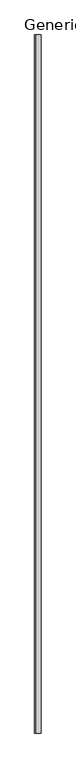
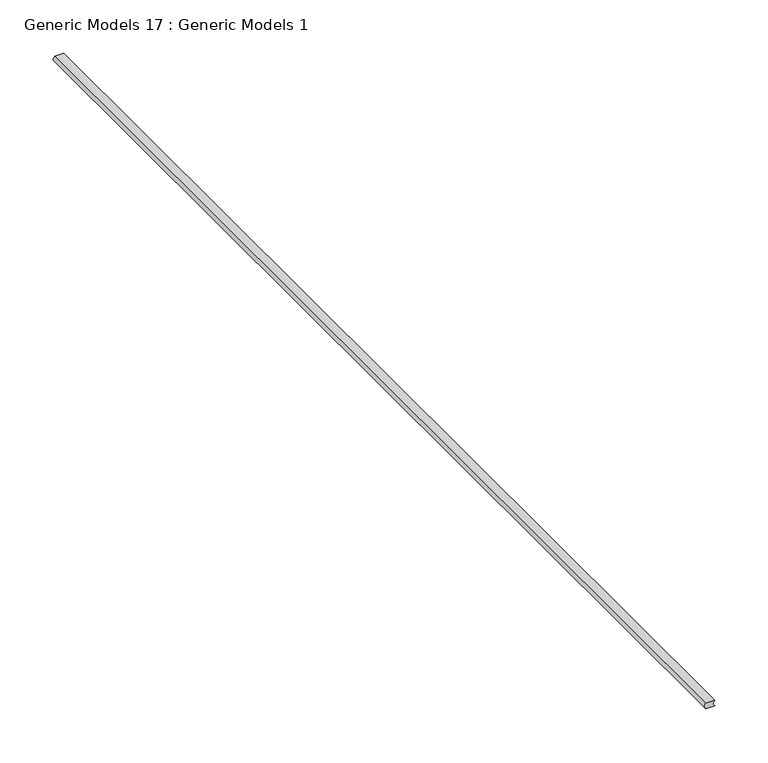
"""IFC4 building model written with IfcOpenShell, lengths in millimetres: proxy geometry, Generic Models 17 : Generic Models 1."""

import ifcopenshell
import ifcopenshell.guid

model = None  # the IFC model being written
_history = None  # IfcOwnerHistory: only IFC2X3 demands one
_inside = {}  # id of a spatial element -> (the spatial element, [elements in it])
_under = {}  # id of a project, library or spatial element -> (it, [spatial elements below it])
_declared = {}  # id of a project -> (the project, [libraries it declares])
_typed = {}  # id of a type object -> (the type object, [elements of that type])
_made_of = {}  # id of a material, layer set ... -> (it, [elements and type objects made of it])


def new_model(schema):
    """Start an empty IFC model of exactly this schema.

    Asked for "IFC4X3", IfcOpenShell would pick the latest addendum, in which some entities
    have other attributes; the version numbers below select the first issue.
    IFC2X3 requires an IfcOwnerHistory on every rooted entity: one is made here for all.
    """
    global model, _history
    if schema == "IFC4X3":
        model = ifcopenshell.file(schema_version=(4, 3, 0, 0))
    else:
        model = ifcopenshell.file(schema=schema)
    _inside.clear()
    _under.clear()
    _declared.clear()
    _typed.clear()
    _made_of.clear()
    _history = None
    if model.schema == "IFC2X3":
        org = make("IfcOrganization", Name="unknown")
        user = make(
            "IfcPersonAndOrganization",
            ThePerson=make("IfcPerson", FamilyName="unknown"),
            TheOrganization=org,
        )
        app = make(
            "IfcApplication",
            ApplicationDeveloper=org,
            Version="unknown",
            ApplicationFullName="unknown",
            ApplicationIdentifier="unknown",
        )
        _history = make(
            "IfcOwnerHistory",
            OwningUser=user,
            OwningApplication=app,
            ChangeAction="ADDED",
            CreationDate=0,
        )
    return model


def make(cls, **values):
    """One entity of the class cls with the attributes given. An attribute that is None is left unset."""
    return model.create_entity(
        cls, **{name: value for name, value in values.items() if value is not None}
    )


def rooted(cls, **values):
    """An entity with a GlobalId (a new one), such as an element, a storey or a relation."""
    return make(cls, GlobalId=ifcopenshell.guid.new(), OwnerHistory=_history, **values)


def si_unit(unit_type, name, prefix=None):
    """IfcSIUnit, for example si_unit("LENGTHUNIT", "METRE", prefix="MILLI")."""
    return make("IfcSIUnit", UnitType=unit_type, Prefix=prefix, Name=name)


def assignment(units):
    """IfcUnitAssignment: the units of a project."""
    return None if units is None else make("IfcUnitAssignment", Units=units)


def point(xyz):
    """IfcCartesianPoint."""
    return None if xyz is None else make("IfcCartesianPoint", Coordinates=xyz)


def direction(xyz):
    """IfcDirection."""
    return None if xyz is None else make("IfcDirection", DirectionRatios=xyz)


def frame(location, z_axis=None, x_axis=None):
    """IfcAxis2Placement3D, a coordinate frame: its origin and axes. An axis left out is left unset."""
    return make(
        "IfcAxis2Placement3D",
        Location=point(location),
        Axis=direction(z_axis),
        RefDirection=direction(x_axis),
    )


def frame_2d(location, x_axis=None):
    """IfcAxis2Placement2D, a coordinate frame in the plane: its origin and x axis."""
    return make(
        "IfcAxis2Placement2D", Location=point(location), RefDirection=direction(x_axis)
    )


def origin():
    """The frame at (0, 0, 0) with its axes left unset."""
    return frame((0.0, 0.0, 0.0))


def place(relative_to, where):
    """IfcLocalPlacement: puts the frame where relative to a parent placement (None: the world)."""
    return make(
        "IfcLocalPlacement", PlacementRelTo=relative_to, RelativePlacement=where
    )


def context(
    kind, dimensions, precision=None, world=None, true_north=None, identifier=None
):
    """IfcGeometricRepresentationContext, for example the 3D "Model" context."""
    return make(
        "IfcGeometricRepresentationContext",
        ContextIdentifier=identifier,
        ContextType=kind,
        CoordinateSpaceDimension=dimensions,
        Precision=precision,
        WorldCoordinateSystem=world,
        TrueNorth=true_north,
    )


def project(units=None, contexts=None):
    """IfcProject with its units and contexts."""
    return rooted(
        "IfcProject",
        Name="project",
        RepresentationContexts=contexts,
        UnitsInContext=assignment(units),
    )


def spatial(cls, under=None, at=None, **own):
    """A site, building, storey or space (cls), placed at a placement, below another one or the project."""
    s = rooted(cls, ObjectPlacement=at, **own)
    if under is not None:
        _under.setdefault(under.id(), (under, []))[1].append(s)
    return s


def polyline(points):
    """IfcPolyline through the points."""
    return make("IfcPolyline", Points=[point(p) for p in points])


def circle_curve(where, radius):
    """IfcCircle in the frame where."""
    return make("IfcCircle", Position=where, Radius=radius)


def trimmed(basis, trim1, trim2, sense, master):
    """IfcTrimmedCurve: the piece of a basis curve between two trims."""
    return make(
        "IfcTrimmedCurve",
        BasisCurve=basis,
        Trim1=trim1,
        Trim2=trim2,
        SenseAgreement=sense,
        MasterRepresentation=master,
    )


def segment(curve, same_sense, transition):
    """IfcCompositeCurveSegment."""
    return make(
        "IfcCompositeCurveSegment",
        Transition=transition,
        SameSense=same_sense,
        ParentCurve=curve,
    )


def composite_curve(segments, self_intersect=None):
    """IfcCompositeCurve: segments joined end to end."""
    return make("IfcCompositeCurve", Segments=segments, SelfIntersect=self_intersect)


def outline(outer, holes=None, kind="AREA"):
    """IfcArbitraryClosedProfileDef: a profile drawn as a closed curve; with holes, ...WithVoids."""
    if holes is None:
        return make("IfcArbitraryClosedProfileDef", ProfileType=kind, OuterCurve=outer)
    return make(
        "IfcArbitraryProfileDefWithVoids",
        ProfileType=kind,
        OuterCurve=outer,
        InnerCurves=holes,
    )


def extrude(swept, where, along, depth):
    """IfcExtrudedAreaSolid: the profile swept, set in the frame where, extruded along a direction by depth."""
    return make(
        "IfcExtrudedAreaSolid",
        SweptArea=swept,
        Position=where,
        ExtrudedDirection=direction(along),
        Depth=depth,
    )


def shape(context_of_items, identifier, shape_type, items):
    """IfcShapeRepresentation: the items that make up one representation, for example the "Body"."""
    return make(
        "IfcShapeRepresentation",
        ContextOfItems=context_of_items,
        RepresentationIdentifier=identifier,
        RepresentationType=shape_type,
        Items=items,
    )


def source(mapping_origin, context_of_items, identifier, shape_type, items):
    """IfcRepresentationMap: a shape defined once, which mapped items show again and again."""
    return make(
        "IfcRepresentationMap",
        MappingOrigin=mapping_origin,
        MappedRepresentation=shape(context_of_items, identifier, shape_type, items),
    )


def transform(
    local_origin,
    x_axis=None,
    y_axis=None,
    z_axis=None,
    scale=None,
    scale2=None,
    scale3=None,
    uniform=True,
):
    """IfcCartesianTransformationOperator3D, or its non-uniform kind. x_axis, y_axis, z_axis: its Axis1, 2, 3."""
    if uniform:
        return make(
            "IfcCartesianTransformationOperator3D",
            Axis1=direction(x_axis),
            Axis2=direction(y_axis),
            LocalOrigin=point(local_origin),
            Scale=scale,
            Axis3=direction(z_axis),
        )
    return make(
        "IfcCartesianTransformationOperator3DnonUniform",
        Axis1=direction(x_axis),
        Axis2=direction(y_axis),
        LocalOrigin=point(local_origin),
        Scale=scale,
        Axis3=direction(z_axis),
        Scale2=scale2,
        Scale3=scale3,
    )


def mapped(mapping_source, mapping_target):
    """IfcMappedItem: shows the shape of a source again, moved by a transform."""
    return make(
        "IfcMappedItem", MappingSource=mapping_source, MappingTarget=mapping_target
    )


def made_of(thing, what):
    """Note that an element or type object is made of a material, layer set ...; save() writes the relation."""
    if what is not None:
        _made_of.setdefault(what.id(), (what, []))[1].append(thing)
    return thing


def element(
    cls,
    number,
    at=None,
    inside=None,
    cuts=None,
    type_object=None,
    material=None,
    context=None,
    identifier="Body",
    shape_type=None,
    held_by="IfcProductDefinitionShape",
    body=None,
    shapes=None,
    **own,
):
    """One element of the class cls, such as IfcWall. Its Tag is "e" and its number.

    at: its placement. inside: the storey or other place that contains it. cuts: it is an
    opening in that element (IfcRelVoidsElement). A single representation is given by context,
    identifier, shape_type and body (its items); several are given by shapes. held_by: the class
    of the entity that holds the representations. save() writes the other relations.
    """
    e = rooted(cls, Tag="e%d" % number, ObjectPlacement=at, **own)
    if body is not None:
        shapes = [shape(context, identifier, shape_type, body)]
    if shapes is not None:
        e.Representation = make(held_by, Representations=shapes)
    if inside is not None:
        _inside.setdefault(inside.id(), (inside, []))[1].append(e)
    if cuts is not None:
        rooted(
            "IfcRelVoidsElement", RelatingBuildingElement=cuts, RelatedOpeningElement=e
        )
    if type_object is not None:
        _typed.setdefault(type_object.id(), (type_object, []))[1].append(e)
    return made_of(e, material)


def aggregate(whole, parts):
    """IfcRelAggregates: a whole, such as a stair, and the parts it consists of."""
    return rooted("IfcRelAggregates", RelatingObject=whole, RelatedObjects=parts)


def save(model, path):
    """Write the relations noted so far, then the file.

    IfcRelAggregates (storeys below a building ...), IfcRelContainedInSpatialStructure (elements
    in a storey), IfcRelDefinesByType, IfcRelAssociatesMaterial and IfcRelDeclares: one each for
    every whole, place, type object, material and project.
    """
    for whole, parts in _under.values():
        aggregate(whole, parts)
    for where, things in _inside.values():
        rooted(
            "IfcRelContainedInSpatialStructure",
            RelatedElements=things,
            RelatingStructure=where,
        )
    for kind, things in _typed.values():
        rooted("IfcRelDefinesByType", RelatedObjects=things, RelatingType=kind)
    for what, things in _made_of.values():
        rooted("IfcRelAssociatesMaterial", RelatedObjects=things, RelatingMaterial=what)
    for by, libraries in _declared.values():
        rooted("IfcRelDeclares", RelatingContext=by, RelatedDefinitions=libraries)
    model.write(path)


def generic_models_17_generic_models_1_e2b33365(model_context):
    return source(origin(), model_context, "Body", "SweptSolid", [
        extrude(outline(composite_curve([segment(trimmed(circle_curve(frame_2d((-1921.2723206, 52669.2343513)), 4.3100275), [point((-1924.4473206, 52666.3196108))], [point((-1918.0973206, 52666.3196108))], True, "CARTESIAN"), True, "CONTINUOUS"), segment(polyline([(-1918.0973206, 52666.3196108), (-1918.0973206, 52656.7946108)]), True, "CONTINUOUS"), segment(trimmed(circle_curve(frame_2d((-1921.2723206, 52659.7093513)), 4.3100275), [point((-1918.0973206, 52656.7946108))], [point((-1924.4473206, 52656.7946108))], False, "CARTESIAN"), True, "CONTINUOUS"), segment(polyline([(-1924.4473206, 52656.7946108), (-1924.4473206, 52666.3196108)]), True, "CONTINUOUS")], self_intersect=False)), frame((0.0, 0.0, 0.0), z_axis=(0.0, 1.0, 0.0), x_axis=(0.0, 0.0, 1.0)), (0.0, 0.0, 1.0), 1219.2),
    ])


if __name__ == "__main__":
    model = new_model("IFC4")
    model_context = context("Model", 3, world=origin())
    ifc_project = project(units=[si_unit("LENGTHUNIT", "METRE", prefix="MILLI")], contexts=[model_context])
    site = spatial("IfcSite", under=ifc_project)
    building = spatial("IfcBuilding", under=site)
    placement = place(None, origin())
    generic_models_17_generic_models_1_shape = generic_models_17_generic_models_1_e2b33365(model_context)
    element("IfcBuildingElementProxy", 1, Name="Generic Models 17 : Generic Models 1", ObjectType="Generic Models 17 : Generic Models 1", at=placement, inside=building, context=model_context, shape_type="MappedRepresentation", body=[
        mapped(generic_models_17_generic_models_1_shape, transform((0.0, 0.0, 0.0), x_axis=(1.0, 0.0, 0.0), y_axis=(0.0, 1.0, 0.0), z_axis=(0.0, 0.0, 1.0))),
    ])
    save(model, "model.ifc")

# Revit data of these elements
# Element 1 (IfcBuildingElementProxy, "Generic Models 17 : Generic Models 1")
#   Materials on its faces: "ACOUSTICAL SEALANT"
# Materials
#   "ACOUSTICAL SEALANT": class "Unassigned", colour RGB 120 120 120, transparency 0, Cost = 0
